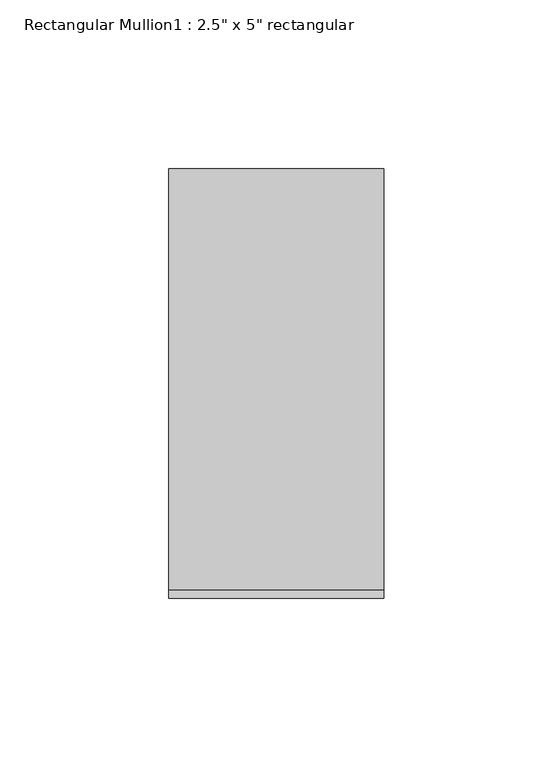
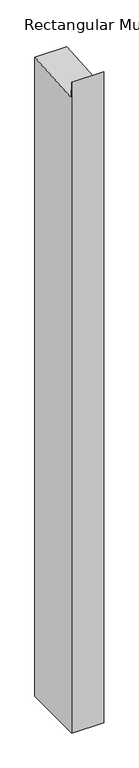
"""IFC4 building model written with IfcOpenShell, lengths in millimetres: member geometry."""

from ifc_helpers import new_model, si_unit, frame, origin, place, context, project, spatial, polyline, outline, extrude, source, transform, mapped, element, save


def member_58fb4e6d(model_context):
    return source(origin(), model_context, "Body", "SweptSolid", [
        extrude(outline(polyline([(-63.5, 29.3948455), (-60.9736199, -4.616608), (63.5, 4.6293267), (63.5, -1339.4207165), (-63.5, -1339.4207165), (-63.5, 29.3948455)])), frame((-63.5, 0.0, 0.0), z_axis=(1.0, 0.0, 0.0), x_axis=(0.0, 1.0, 0.0)), (0.0, 0.0, 1.0), 63.5),
    ])


if __name__ == "__main__":
    model = new_model("IFC4")
    model_context = context("Model", 3, world=origin())
    ifc_project = project(units=[si_unit("LENGTHUNIT", "METRE", prefix="MILLI")], contexts=[model_context])
    site = spatial("IfcSite", under=ifc_project)
    building = spatial("IfcBuilding", under=site)
    placement = place(None, origin())
    member_shape = member_58fb4e6d(model_context)
    element("IfcMember", 1, ObjectType="Rectangular Mullion1 : 2.5\" x 5\" rectangular", at=placement, inside=building, context=model_context, shape_type="MappedRepresentation", body=[
        mapped(member_shape, transform((0.0, 0.0, 0.0), x_axis=(1.0, 0.0, 0.0), y_axis=(0.0, 1.0, 0.0), z_axis=(0.0, 0.0, 1.0))),
    ])
    save(model, "model.ifc")

# Revit data of these elements
# Type "Rectangular Mullion1 : 2.5\" x 5\" rectangular"
#   built-in parameter 1007304 = 0.416667 (stored number, unit not read)
#   built-in parameter 1007301 = 0.104167 (stored number, unit not read)
#   built-in parameter 1007300 = 0.104167 (stored number, unit not read)
# Element 1 (IfcMember, "Rectangular Mullion1 : 2.5\" x 5\" rectangular")
#   Materials on its faces: "support-frame"
# Materials
#   "support-frame": class "Unassigned", colour RGB 233 233 233, transparency 0, Cost = 0
